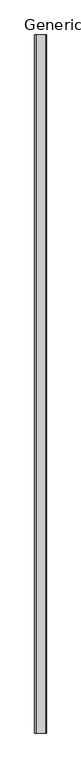
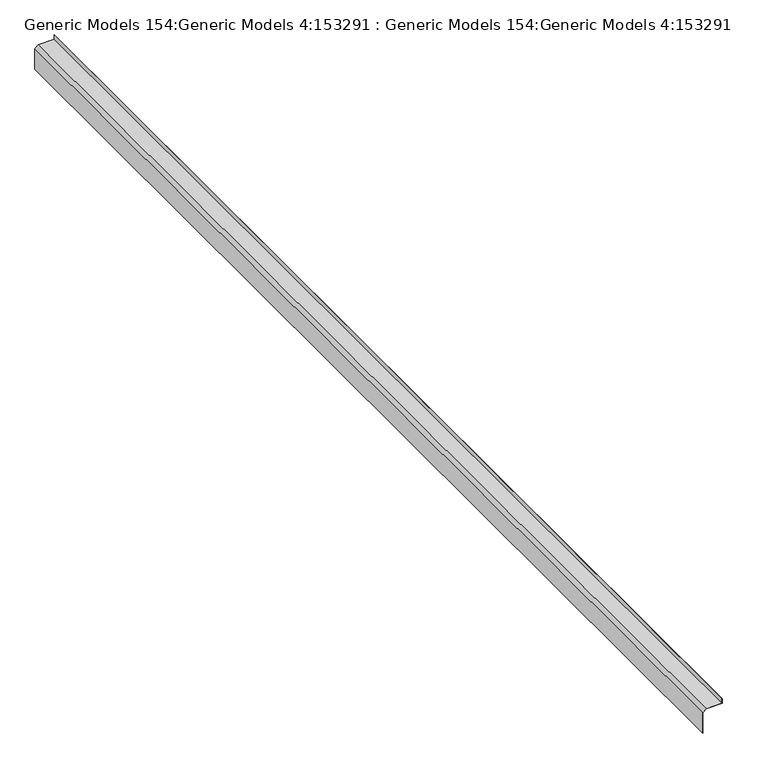
"""IFC4 building model written with IfcOpenShell, lengths in millimetres: proxy geometry, Generic Models 154:Generic Models 4:153291 : Generic Models 154:Generic Models 4:153291."""

from ifc_helpers import new_model, si_unit, frame, origin, place, context, project, spatial, polyline, outline, extrude, source, transform, mapped, element, save


def generic_models_154_generic_models_4_153291_generic_models_6df6a242(model_context):
    return source(origin(), model_context, "Body", "SweptSolid", [
        extrude(outline(polyline([(-35.2872651, -6651.0686422), (-35.2872651, -6542.1569949), (-2.7435151, -6542.1569949), (-2.7435151, -6542.9507449), (-34.4935151, -6542.9507449), (-34.4935151, -6651.3974242), (-56.6153733, -6673.5192825), (-202.9941554, -6673.5192825), (-202.9941554, -6672.7255325), (-56.9441554, -6672.7255325), (-35.2872651, -6651.0686422)])), frame((0.0, -5303.1974793, 0.0), z_axis=(0.0, 1.0, 0.0), x_axis=(0.0, 0.0, 1.0)), (0.0, 0.0, 1.0), 7886.7),
    ])


if __name__ == "__main__":
    model = new_model("IFC4")
    model_context = context("Model", 3, world=origin())
    ifc_project = project(units=[si_unit("LENGTHUNIT", "METRE", prefix="MILLI")], contexts=[model_context])
    site = spatial("IfcSite", under=ifc_project)
    building = spatial("IfcBuilding", under=site)
    placement = place(None, origin())
    generic_models_154_generic_models_4_153291_generic_models_shape = generic_models_154_generic_models_4_153291_generic_models_6df6a242(model_context)
    element("IfcBuildingElementProxy", 1, Name="Generic Models 154:Generic Models 4:153291 : Generic Models 154:Generic Models 4:153291", ObjectType="Generic Models 154:Generic Models 4:153291 : Generic Models 154:Generic Models 4:153291", at=placement, inside=building, context=model_context, shape_type="MappedRepresentation", body=[
        mapped(generic_models_154_generic_models_4_153291_generic_models_shape, transform((0.0, 0.0, 0.0), x_axis=(1.0, 0.0, 0.0), y_axis=(0.0, 1.0, 0.0), z_axis=(0.0, 0.0, 1.0))),
    ])
    save(model, "model.ifc")

# Revit data of these elements
# Type "Generic Models 154:Generic Models 4:153291 : Generic Models 154:Generic Models 4:153291"
#   NameOverride = "Generic Models 154:Generic Models 4:153291"
#   ObjectTypeOverride = "Generic Models 154:Generic Models 4"
#   Reference = "Generic Models 4"
#   Category = "Generic Models"
#   Tag = "153291"
# Element 1 (IfcBuildingElementProxy, "Generic Models 154:Generic Models 4:153291 : Generic Models 154:Generic Models 4:153291")
#   Materials on its faces: "_16 GA. COPPER BRAKE METAL FLASHING W/ END DAMS 12508"
# Materials
#   "_16 GA. COPPER BRAKE METAL FLASHING W/ END DAMS 12508": class "Unassigned", colour RGB 175 175 175, transparency 0
